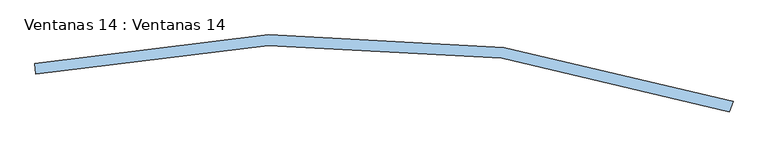
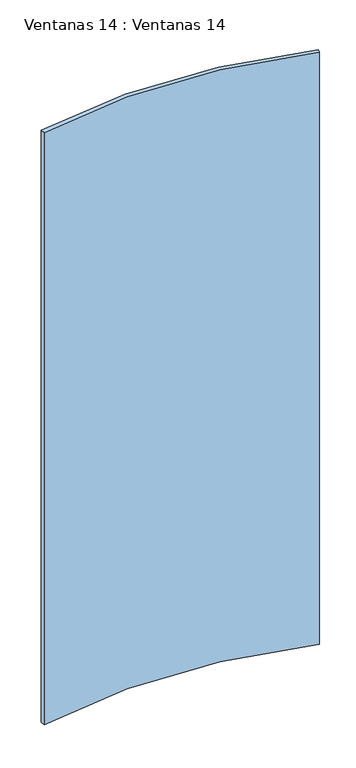
"""IFC4 building model written with IfcOpenShell, lengths in millimetres: window geometry, Ventanas 14 : Ventanas 14."""

from ifc_helpers import new_model, si_unit, point, frame, frame_2d, origin, place, context, project, spatial, polyline, circle_curve, trimmed, segment, composite_curve, outline, extrude, source, transform, mapped, element, save


def ventanas_14_ventanas_14_62a1553d(model_context):
    return source(origin(), model_context, "Body", "SweptSolid", [
        extrude(outline(composite_curve([segment(polyline([(-5731.3032904, -84.1518368), (-5738.1436932, -102.9456892)]), True, "CONTINUOUS"), segment(trimmed(circle_curve(frame_2d((-6505.889295, -2418.5153987)), 2439.5279028), [point((-5738.1436932, -102.9456892))], [point((-7019.1736429, -33.5970422))], True, "CARTESIAN"), True, "CONTINUOUS"), segment(polyline([(-7019.1736429, -33.5970422), (-7021.1795689, -13.69789)]), True, "CONTINUOUS"), segment(trimmed(circle_curve(frame_2d((-6505.6154013, -2417.5134903)), 2458.4824285), [point((-7021.1795689, -13.69789))], [point((-5731.3032904, -84.1518368))], False, "CARTESIAN"), True, "CONTINUOUS")], self_intersect=False)), frame((0.0, 0.0, 6100.0), z_axis=(0.0, 0.0, 1.0), x_axis=(1.0, 0.0, 0.0)), (0.0, 0.0, 1.0), 3000.0),
    ])


if __name__ == "__main__":
    model = new_model("IFC4")
    model_context = context("Model", 3, world=origin())
    ifc_project = project(units=[si_unit("LENGTHUNIT", "METRE", prefix="MILLI")], contexts=[model_context])
    site = spatial("IfcSite", under=ifc_project)
    building = spatial("IfcBuilding", under=site)
    placement = place(None, origin())
    ventanas_14_ventanas_14_shape = ventanas_14_ventanas_14_62a1553d(model_context)
    element("IfcWindow", 1, ObjectType="Ventanas 14 : Ventanas 14", at=placement, inside=building, context=model_context, shape_type="MappedRepresentation", body=[
        mapped(ventanas_14_ventanas_14_shape, transform((0.0, 0.0, 0.0), x_axis=(1.0, 0.0, 0.0), y_axis=(0.0, 1.0, 0.0), z_axis=(0.0, 0.0, 1.0))),
    ])
    save(model, "model.ifc")

# Revit data of these elements
# Type "Ventanas 14 : Ventanas 14"
#   Type Mark = "40"
# Element 1 (IfcWindow, "Ventanas 14 : Ventanas 14")
#   Materials on its faces: "VIDRIO"
# Materials
#   "VIDRIO": class "Genérico", colour RGB 120 120 120, transparency 0, Cost = 0
